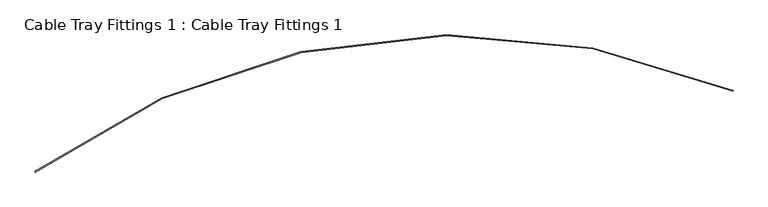
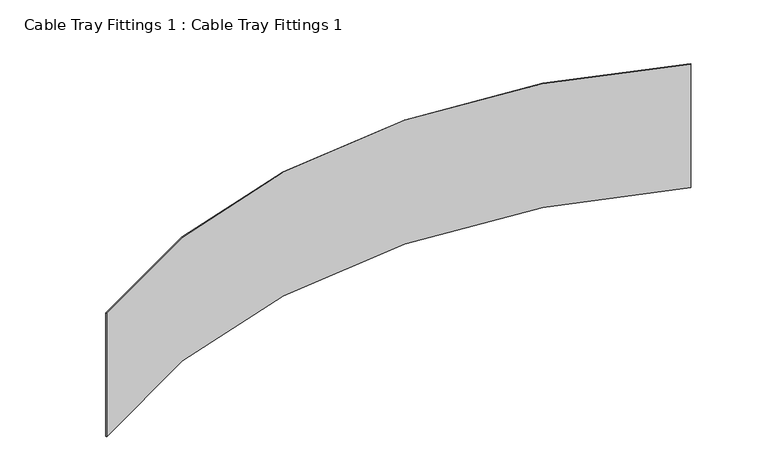
"""IFC4 building model written with IfcOpenShell, lengths in millimetres: furniture geometry, Cable Tray Fittings 1 : Cable Tray Fittings 1."""

from ifc_helpers import new_model, si_unit, point, frame, frame_2d, origin, place, context, project, spatial, polyline, circle_curve, trimmed, segment, composite_curve, outline, extrude, source, transform, mapped, element, save


def cable_tray_fittings_1_cable_tray_fittings_1_77ebdb05(model_context):
    return source(origin(), model_context, "Body", "SweptSolid", [
        extrude(outline(composite_curve([segment(polyline([(-2594.907124, -22719.5323335), (-2596.7150951, -22716.9212916)]), True, "CONTINUOUS"), segment(trimmed(circle_curve(frame_2d((-836.3775196, -25134.6312821)), 2990.6704897), [point((-2596.7150951, -22716.9212916))], [point((322.1462255, -22377.4710201))], False, "CARTESIAN"), True, "CONTINUOUS"), segment(polyline([(322.1462255, -22377.4710201), (321.0078502, -22380.4365891)]), True, "CONTINUOUS"), segment(trimmed(circle_curve(frame_2d((-836.3775196, -25134.6312821)), 2987.4954897), [point((321.0078502, -22380.4365891))], [point((-2594.907124, -22719.5323335))], True, "CARTESIAN"), True, "CONTINUOUS")], self_intersect=False)), frame((0.0, 0.0, 371.475), z_axis=(0.0, 0.0, 1.0), x_axis=(1.0, 0.0, 0.0)), (0.0, 0.0, 1.0), 609.6),
    ])


if __name__ == "__main__":
    model = new_model("IFC4")
    model_context = context("Model", 3, world=origin())
    ifc_project = project(units=[si_unit("LENGTHUNIT", "METRE", prefix="MILLI")], contexts=[model_context])
    site = spatial("IfcSite", under=ifc_project)
    building = spatial("IfcBuilding", under=site)
    placement = place(None, origin())
    cable_tray_fittings_1_cable_tray_fittings_1_shape = cable_tray_fittings_1_cable_tray_fittings_1_77ebdb05(model_context)
    element("IfcFurniture", 1, ObjectType="Cable Tray Fittings 1 : Cable Tray Fittings 1", at=placement, inside=building, context=model_context, shape_type="MappedRepresentation", body=[
        mapped(cable_tray_fittings_1_cable_tray_fittings_1_shape, transform((0.0, 0.0, 0.0), x_axis=(1.0, 0.0, 0.0), y_axis=(0.0, 1.0, 0.0), z_axis=(0.0, 0.0, 1.0))),
    ])
    save(model, "model.ifc")

# Revit data of these elements
# Element 1 (IfcFurniture, "Cable Tray Fittings 1 : Cable Tray Fittings 1")
#   Materials on its faces: "PERFORATED METAL"
# Materials
#   "PERFORATED METAL": class "Generic", colour RGB 230 230 230, transparency 0, Cost = 0
